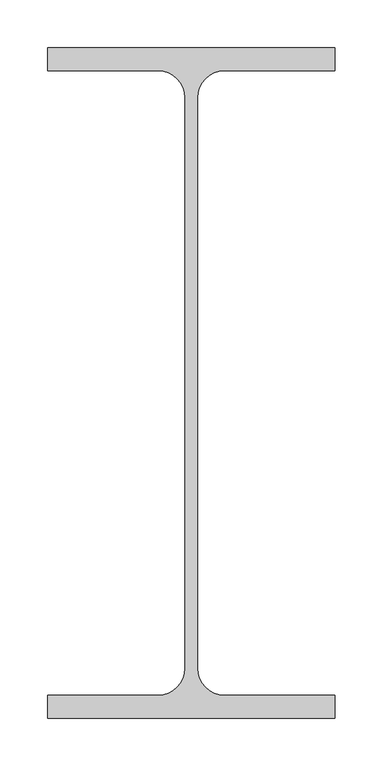
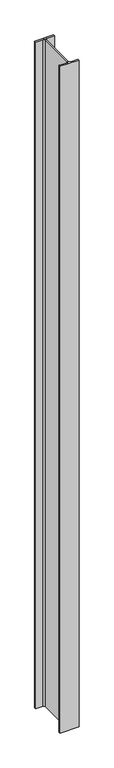
"""IFC4 building model written with IfcOpenShell, lengths in millimetres: column geometry, 0912_Steel Column_H_KSD3502 : H_SC_ASC_H-700x300x13x24."""

from ifc_helpers import new_model, si_unit, point, frame, frame_2d, origin, place, context, project, spatial, polyline, circle_curve, trimmed, segment, composite_curve, outline, extrude, source, transform, mapped, element, save


def column_8461dad7(model_context):
    return source(origin(), model_context, "Body", "SweptSolid", [
        extrude(outline(composite_curve([segment(polyline([(150.0, 350.0), (150.0, 326.0), (34.5, 326.0)]), True, "CONTINUOUS"), segment(trimmed(circle_curve(frame_2d((34.5, 298.0)), 28.0), [point((34.5, 326.0))], [point((6.5, 298.0))], True, "CARTESIAN"), True, "CONTINUOUS"), segment(polyline([(6.5, 298.0), (6.5, -298.0)]), True, "CONTINUOUS"), segment(trimmed(circle_curve(frame_2d((34.5, -298.0)), 28.0), [point((6.5, -298.0))], [point((34.5, -326.0))], True, "CARTESIAN"), True, "CONTINUOUS"), segment(polyline([(34.5, -326.0), (150.0, -326.0), (150.0, -350.0), (-150.0, -350.0), (-150.0, -326.0), (-34.5, -326.0)]), True, "CONTINUOUS"), segment(trimmed(circle_curve(frame_2d((-34.5, -298.0)), 28.0), [point((-34.5, -326.0))], [point((-6.5, -298.0))], True, "CARTESIAN"), True, "CONTINUOUS"), segment(polyline([(-6.5, -298.0), (-6.5, 298.0)]), True, "CONTINUOUS"), segment(trimmed(circle_curve(frame_2d((-34.5, 298.0)), 28.0), [point((-6.5, 298.0))], [point((-34.5, 326.0))], True, "CARTESIAN"), True, "CONTINUOUS"), segment(polyline([(-34.5, 326.0), (-150.0, 326.0), (-150.0, 350.0), (150.0, 350.0)]), True, "CONTINUOUS")], self_intersect=False)), frame((0.0, 0.0, 685.9720055), z_axis=(0.0, 0.0, 1.0), x_axis=(1.0, 0.0, 0.0)), (0.0, 0.0, 1.0), 11224.0),
    ])


if __name__ == "__main__":
    model = new_model("IFC4")
    model_context = context("Model", 3, world=origin())
    ifc_project = project(units=[si_unit("LENGTHUNIT", "METRE", prefix="MILLI")], contexts=[model_context])
    site = spatial("IfcSite", under=ifc_project)
    building = spatial("IfcBuilding", under=site)
    placement = place(None, origin())
    column_shape = column_8461dad7(model_context)
    element("IfcColumn", 1, ObjectType="0912_Steel Column_H_KSD3502 : H_SC_ASC_H-700x300x13x24", at=placement, inside=building, context=model_context, shape_type="MappedRepresentation", body=[
        mapped(column_shape, transform((0.0, 0.0, 0.0), x_axis=(1.0, 0.0, 0.0), y_axis=(0.0, 1.0, 0.0), z_axis=(0.0, 0.0, 1.0))),
    ])
    save(model, "model.ifc")

# Revit data of these elements
# Type "0912_Steel Column_H_KSD3502 : H_SC_ASC_H-700x300x13x24"
#   H_WM Code_1 = "S01AA002-00001 | Main Steel Structure Fabrication Work | Shelter/Building | Medium Steel - Standard (90KG/M>Weight≥30KG/M) | Material: (   )"
#   H_WM Code_2 = "S03AA028-00001 | Main Steel Structure Erection Work | Shelter/Building | Medium Steel (90KG/M>Weight≥30KG/M) | Material: (   )"
#   H_WM Code_3 = "S01AA010-00001 | Main Steel Structure Fabrication Work | Shelter/Building | Steel Painting/Coating | for Non-Fireproofed Steel Surface, Surface Preparation, Primer, Second & Final Coat | Material: (   )"
#   H_Q'ty Cal Type Tag = "SC-Q2"
#   Width = 30.0 cm
#   Web Thickness = 1.3 cm
#   Web Fillet = 2.8 cm
#   Warping Constant = 12338400.0 cm⁶
#   Torsional Moment of Inertia = 325.986 cm⁴
#   Section Area = 235.5 cm²
#   Plastic Modulus weak axis = 1120.0 cm³
#   Plastic Modulus strong axis = 6460.0 cm³
#   Perimeter = 2.53 m²/m
#   Nominal Weight = 185.00 kgf/m
#   Moment of Inertia weak axis = 10800.00 cm⁴
#   Moment of Inertia strong axis = 201000.00 cm⁴
#   Height = 70.0 cm
#   Flange Thickness = 2.4 cm
#   Elastic Modulus weak axis = 722.0 cm³
#   Elastic Modulus strong axis = 5760.0 cm³
#   Centroid Vertical = 35.0 cm
#   Centroid Horizontal = 15.0 cm
#   Structural Material [instance default] = Steel, 45-345
#   Section Name Key = ""
#   Bolt Spacing = 0
#   Assembly Code = ""
# Element 1 (IfcColumn, "0912_Steel Column_H_KSD3502 : H_SC_ASC_H-700x300x13x24")
#   Structural Material = A03AD029-00008_Anchor Bolt (Installation only)_M36
#   Materials on its faces: "A03AD029-00008_Anchor Bolt (Installation only)_M36"
# Materials
#   "Steel, 45-345": class "Metal", colour RGB 189 187 185, transparency 0, Description = "Steel 345 MPa", Cost = 0
#   "A03AD029-00008_Anchor Bolt (Installation only)_M36": class "Unassigned", colour RGB 84 83 81, transparency 0, Cost = 0
